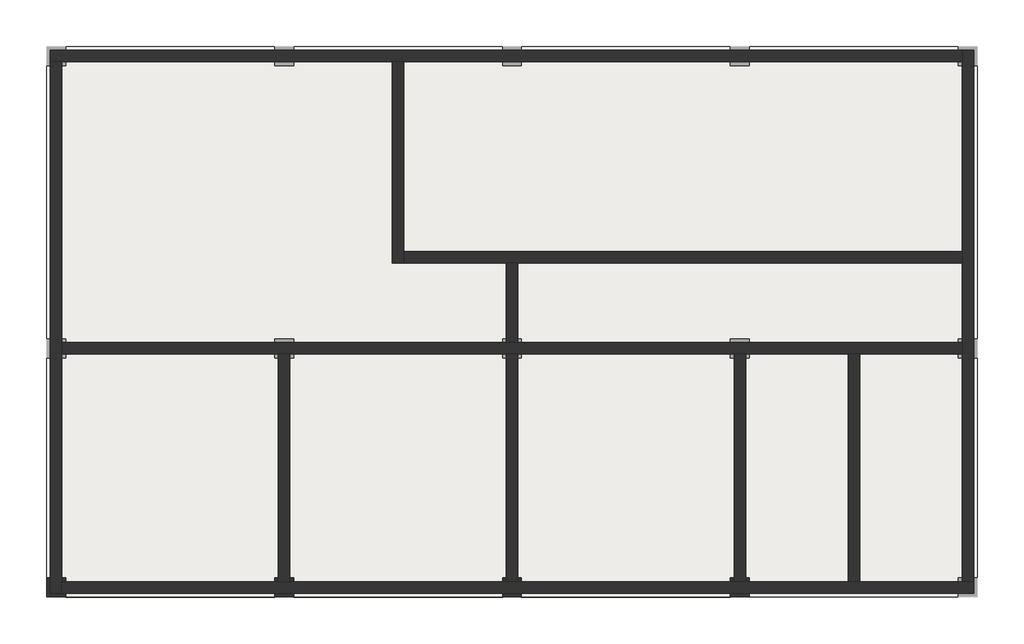
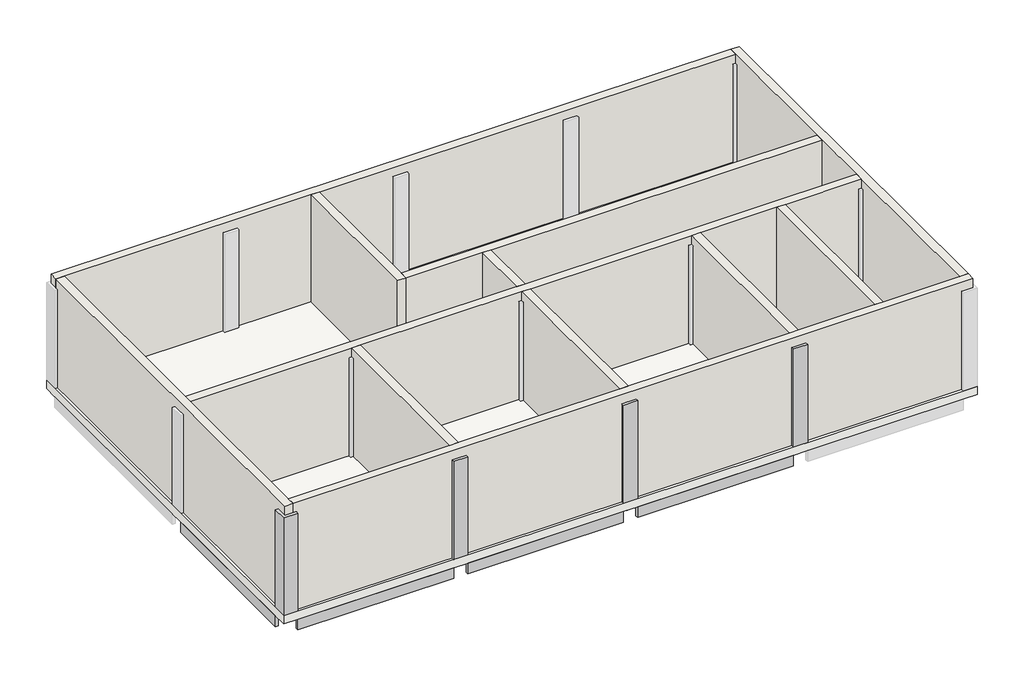
# One storey, part 1 of 2: 12 walls, 7 beams, 4 columns, 1 slab.
"""IFC4 building model written with IfcOpenShell, lengths in millimetres."""

import ifcopenshell
import ifcopenshell.guid

model = None  # the IFC model being written
_history = None  # IfcOwnerHistory: only IFC2X3 demands one
_inside = {}  # id of a spatial element -> (the spatial element, [elements in it])
_under = {}  # id of a project, library or spatial element -> (it, [spatial elements below it])
_declared = {}  # id of a project -> (the project, [libraries it declares])
_typed = {}  # id of a type object -> (the type object, [elements of that type])
_made_of = {}  # id of a material, layer set ... -> (it, [elements and type objects made of it])


def new_model(schema):
    """Start an empty IFC model of exactly this schema.

    Asked for "IFC4X3", IfcOpenShell would pick the latest addendum, in which some entities
    have other attributes; the version numbers below select the first issue.
    IFC2X3 requires an IfcOwnerHistory on every rooted entity: one is made here for all.
    """
    global model, _history
    if schema == "IFC4X3":
        model = ifcopenshell.file(schema_version=(4, 3, 0, 0))
    else:
        model = ifcopenshell.file(schema=schema)
    _inside.clear()
    _under.clear()
    _declared.clear()
    _typed.clear()
    _made_of.clear()
    _history = None
    if model.schema == "IFC2X3":
        org = make("IfcOrganization", Name="unknown")
        user = make(
            "IfcPersonAndOrganization",
            ThePerson=make("IfcPerson", FamilyName="unknown"),
            TheOrganization=org,
        )
        app = make(
            "IfcApplication",
            ApplicationDeveloper=org,
            Version="unknown",
            ApplicationFullName="unknown",
            ApplicationIdentifier="unknown",
        )
        _history = make(
            "IfcOwnerHistory",
            OwningUser=user,
            OwningApplication=app,
            ChangeAction="ADDED",
            CreationDate=0,
        )
    return model


def make(cls, **values):
    """One entity of the class cls with the attributes given. An attribute that is None is left unset."""
    return model.create_entity(
        cls, **{name: value for name, value in values.items() if value is not None}
    )


def rooted(cls, **values):
    """An entity with a GlobalId (a new one), such as an element, a storey or a relation."""
    return make(cls, GlobalId=ifcopenshell.guid.new(), OwnerHistory=_history, **values)


def si_unit(unit_type, name, prefix=None):
    """IfcSIUnit, for example si_unit("LENGTHUNIT", "METRE", prefix="MILLI")."""
    return make("IfcSIUnit", UnitType=unit_type, Prefix=prefix, Name=name)


def assignment(units):
    """IfcUnitAssignment: the units of a project."""
    return None if units is None else make("IfcUnitAssignment", Units=units)


def point(xyz):
    """IfcCartesianPoint."""
    return None if xyz is None else make("IfcCartesianPoint", Coordinates=xyz)


def direction(xyz):
    """IfcDirection."""
    return None if xyz is None else make("IfcDirection", DirectionRatios=xyz)


def frame(location, z_axis=None, x_axis=None):
    """IfcAxis2Placement3D, a coordinate frame: its origin and axes. An axis left out is left unset."""
    return make(
        "IfcAxis2Placement3D",
        Location=point(location),
        Axis=direction(z_axis),
        RefDirection=direction(x_axis),
    )


def origin():
    """The frame at (0, 0, 0) with its axes left unset."""
    return frame((0.0, 0.0, 0.0))


def place(relative_to, where):
    """IfcLocalPlacement: puts the frame where relative to a parent placement (None: the world)."""
    return make(
        "IfcLocalPlacement", PlacementRelTo=relative_to, RelativePlacement=where
    )


def context(
    kind, dimensions, precision=None, world=None, true_north=None, identifier=None
):
    """IfcGeometricRepresentationContext, for example the 3D "Model" context."""
    return make(
        "IfcGeometricRepresentationContext",
        ContextIdentifier=identifier,
        ContextType=kind,
        CoordinateSpaceDimension=dimensions,
        Precision=precision,
        WorldCoordinateSystem=world,
        TrueNorth=true_north,
    )


def project(units=None, contexts=None):
    """IfcProject with its units and contexts."""
    return rooted(
        "IfcProject",
        Name="project",
        RepresentationContexts=contexts,
        UnitsInContext=assignment(units),
    )


def spatial(cls, under=None, at=None, **own):
    """A site, building, storey or space (cls), placed at a placement, below another one or the project."""
    s = rooted(cls, ObjectPlacement=at, **own)
    if under is not None:
        _under.setdefault(under.id(), (under, []))[1].append(s)
    return s


def polyline(points):
    """IfcPolyline through the points."""
    return make("IfcPolyline", Points=[point(p) for p in points])


def outline(outer, holes=None, kind="AREA"):
    """IfcArbitraryClosedProfileDef: a profile drawn as a closed curve; with holes, ...WithVoids."""
    if holes is None:
        return make("IfcArbitraryClosedProfileDef", ProfileType=kind, OuterCurve=outer)
    return make(
        "IfcArbitraryProfileDefWithVoids",
        ProfileType=kind,
        OuterCurve=outer,
        InnerCurves=holes,
    )


def extrude(swept, where, along, depth):
    """IfcExtrudedAreaSolid: the profile swept, set in the frame where, extruded along a direction by depth."""
    return make(
        "IfcExtrudedAreaSolid",
        SweptArea=swept,
        Position=where,
        ExtrudedDirection=direction(along),
        Depth=depth,
    )


def faces_of(points, faces, orient=None, outer=None):
    """IfcFace entities. A face is a list of loops; a loop is a list of indices into points, from 0.

    orient and outer hold one flag for each loop. By default every Orientation is true, the
    first loop of a face is its IfcFaceOuterBound and the others are IfcFaceBound.
    """
    made = []
    for i, loops in enumerate(faces):
        bounds = []
        for j, loop in enumerate(loops):
            is_outer = j == 0 if outer is None else outer[i][j]
            bounds.append(
                make(
                    "IfcFaceOuterBound" if is_outer else "IfcFaceBound",
                    Bound=make("IfcPolyLoop", Polygon=[points[k] for k in loop]),
                    Orientation=True if orient is None else orient[i][j],
                )
            )
        made.append(make("IfcFace", Bounds=bounds))
    return made


def faceted_brep(points, faces, orient=None, outer=None, voids=None):
    """IfcFacetedBrep: a solid bounded by flat faces; with voids (closed shells), ...WithVoids."""
    shared = [point(p) for p in points]
    hull = make("IfcClosedShell", CfsFaces=faces_of(shared, faces, orient, outer))
    if voids is None:
        return make("IfcFacetedBrep", Outer=hull)
    return make(
        "IfcFacetedBrepWithVoids",
        Outer=hull,
        Voids=[
            make(cls, CfsFaces=faces_of(shared, fs, o, b)) for cls, fs, o, b in voids
        ],
    )


def shape(context_of_items, identifier, shape_type, items):
    """IfcShapeRepresentation: the items that make up one representation, for example the "Body"."""
    return make(
        "IfcShapeRepresentation",
        ContextOfItems=context_of_items,
        RepresentationIdentifier=identifier,
        RepresentationType=shape_type,
        Items=items,
    )


def made_of(thing, what):
    """Note that an element or type object is made of a material, layer set ...; save() writes the relation."""
    if what is not None:
        _made_of.setdefault(what.id(), (what, []))[1].append(thing)
    return thing


def element(
    cls,
    number,
    at=None,
    inside=None,
    cuts=None,
    type_object=None,
    material=None,
    context=None,
    identifier="Body",
    shape_type=None,
    held_by="IfcProductDefinitionShape",
    body=None,
    shapes=None,
    **own,
):
    """One element of the class cls, such as IfcWall. Its Tag is "e" and its number.

    at: its placement. inside: the storey or other place that contains it. cuts: it is an
    opening in that element (IfcRelVoidsElement). A single representation is given by context,
    identifier, shape_type and body (its items); several are given by shapes. held_by: the class
    of the entity that holds the representations. save() writes the other relations.
    """
    e = rooted(cls, Tag="e%d" % number, ObjectPlacement=at, **own)
    if body is not None:
        shapes = [shape(context, identifier, shape_type, body)]
    if shapes is not None:
        e.Representation = make(held_by, Representations=shapes)
    if inside is not None:
        _inside.setdefault(inside.id(), (inside, []))[1].append(e)
    if cuts is not None:
        rooted(
            "IfcRelVoidsElement", RelatingBuildingElement=cuts, RelatedOpeningElement=e
        )
    if type_object is not None:
        _typed.setdefault(type_object.id(), (type_object, []))[1].append(e)
    return made_of(e, material)


def aggregate(whole, parts):
    """IfcRelAggregates: a whole, such as a stair, and the parts it consists of."""
    return rooted("IfcRelAggregates", RelatingObject=whole, RelatedObjects=parts)


def save(model, path):
    """Write the relations noted so far, then the file.

    IfcRelAggregates (storeys below a building ...), IfcRelContainedInSpatialStructure (elements
    in a storey), IfcRelDefinesByType, IfcRelAssociatesMaterial and IfcRelDeclares: one each for
    every whole, place, type object, material and project.
    """
    for whole, parts in _under.values():
        aggregate(whole, parts)
    for where, things in _inside.values():
        rooted(
            "IfcRelContainedInSpatialStructure",
            RelatedElements=things,
            RelatingStructure=where,
        )
    for kind, things in _typed.values():
        rooted("IfcRelDefinesByType", RelatedObjects=things, RelatingType=kind)
    for what, things in _made_of.values():
        rooted("IfcRelAssociatesMaterial", RelatedObjects=things, RelatingMaterial=what)
    for by, libraries in _declared.values():
        rooted("IfcRelDeclares", RelatingContext=by, RelatedDefinitions=libraries)
    model.write(path)


model = new_model("IFC4")

# Units and contexts
model_context = context("Model", 3, world=origin())
ifc_project = project(units=[si_unit("LENGTHUNIT", "METRE", prefix="MILLI")], contexts=[model_context])

# Site, building, storey
site = spatial("IfcSite", under=ifc_project)
building = spatial("IfcBuilding", under=site)
storey = spatial("IfcBuildingStorey", under=building, Name="2nd FL GL+6,200", Elevation=6000.0)

# Beams
placement = place(None, origin())
element("IfcBeam", 1, ObjectType="RC Beam_Rectangular : 350 x 700mm", at=placement, inside=storey, context=model_context, shape_type="SweptSolid", body=[
    extrude(outline(polyline([(-18945.7273237, -4314.0236875), (-18945.7273237, 1485.9763125), (-18845.7273237, 1485.9763125), (-18845.7273237, -4314.0236875), (-18945.7273237, -4314.0236875)])), frame((0.0, 0.0, 5300.0), z_axis=(0.0, 0.0, 1.0), x_axis=(1.0, 0.0, 0.0)), (0.0, 0.0, 1.0), 400.0),
])
element("IfcBeam", 2, ObjectType="RC Beam_Rectangular : 350 x 700mm", at=placement, inside=storey, context=model_context, shape_type="SweptSolid", body=[
    extrude(outline(polyline([(-12520.7273237, 1485.9763125), (-12520.7273237, -4314.0236875), (-12545.7273237, -4314.0236875), (-12545.7273237, 1485.9763125), (-12520.7273237, 1485.9763125)])), frame((0.0, 0.0, 5300.0), z_axis=(0.0, 0.0, 1.0), x_axis=(1.0, 0.0, 0.0)), (0.0, 0.0, 1.0), 400.0),
    extrude(outline(polyline([(-12870.7273237, -4314.0236875), (-12870.7273237, 1485.9763125), (-12845.7273237, 1485.9763125), (-12845.7273237, -4314.0236875), (-12870.7273237, -4314.0236875)])), frame((0.0, 0.0, 5300.0), z_axis=(0.0, 0.0, 1.0), x_axis=(1.0, 0.0, 0.0)), (0.0, 0.0, 1.0), 400.0),
])
element("IfcBeam", 3, ObjectType="RC Beam_Rectangular : 350 x 700mm", at=placement, inside=storey, context=model_context, shape_type="SweptSolid", body=[
    extrude(outline(polyline([(-6520.7273237, 1485.9763125), (-6520.7273237, -4314.0236875), (-6545.7273237, -4314.0236875), (-6545.7273237, 1485.9763125), (-6520.7273237, 1485.9763125)])), frame((0.0, 0.0, 5300.0), z_axis=(0.0, 0.0, 1.0), x_axis=(1.0, 0.0, 0.0)), (0.0, 0.0, 1.0), 400.0),
    extrude(outline(polyline([(-6870.7273237, -4314.0236875), (-6870.7273237, 1485.9763125), (-6845.7273237, 1485.9763125), (-6845.7273237, -4314.0236875), (-6870.7273237, -4314.0236875)])), frame((0.0, 0.0, 5300.0), z_axis=(0.0, 0.0, 1.0), x_axis=(1.0, 0.0, 0.0)), (0.0, 0.0, 1.0), 400.0),
])
element("IfcBeam", 4, ObjectType="RC Beam_Rectangular : 350 x 700mm", at=placement, inside=storey, context=model_context, shape_type="SweptSolid", body=[
    extrude(outline(polyline([(-520.7273237, 1485.9763125), (-520.7273237, -4314.0236875), (-545.7273237, -4314.0236875), (-545.7273237, 1485.9763125), (-520.7273237, 1485.9763125)])), frame((0.0, 0.0, 5300.0), z_axis=(0.0, 0.0, 1.0), x_axis=(1.0, 0.0, 0.0)), (0.0, 0.0, 1.0), 400.0),
    extrude(outline(polyline([(-870.7273237, -4314.0236875), (-870.7273237, 1485.9763125), (-845.7273237, 1485.9763125), (-845.7273237, -4314.0236875), (-870.7273237, -4314.0236875)])), frame((0.0, 0.0, 5300.0), z_axis=(0.0, 0.0, 1.0), x_axis=(1.0, 0.0, 0.0)), (0.0, 0.0, 1.0), 400.0),
])
element("IfcBeam", 5, ObjectType="RC Beam_Rectangular : 350 x 700mm", at=placement, inside=storey, context=model_context, shape_type="SweptSolid", body=[
    extrude(outline(polyline([(-12945.7273237, -4814.0236875), (-18445.7273237, -4814.0236875), (-18445.7273237, -4714.0236875), (-12945.7273237, -4714.0236875), (-12945.7273237, -4814.0236875)])), frame((0.0, 0.0, 5300.0), z_axis=(0.0, 0.0, 1.0), x_axis=(1.0, 0.0, 0.0)), (0.0, 0.0, 1.0), 400.0),
])
element("IfcBeam", 6, ObjectType="RC Beam_Rectangular : 350 x 700mm", at=placement, inside=storey, context=model_context, shape_type="SweptSolid", body=[
    extrude(outline(polyline([(-6945.7273237, -4714.0236875), (-6945.7273237, -4814.0236875), (-12445.7273237, -4814.0236875), (-12445.7273237, -4714.0236875), (-6945.7273237, -4714.0236875)])), frame((0.0, 0.0, 5300.0), z_axis=(0.0, 0.0, 1.0), x_axis=(1.0, 0.0, 0.0)), (0.0, 0.0, 1.0), 400.0),
])
element("IfcBeam", 7, ObjectType="RC Beam_Rectangular : 350 x 700mm", at=placement, inside=storey, context=model_context, shape_type="SweptSolid", body=[
    extrude(outline(polyline([(-945.7273237, -4714.0236875), (-945.7273237, -4814.0236875), (-6445.7273237, -4814.0236875), (-6445.7273237, -4714.0236875), (-945.7273237, -4714.0236875)])), frame((0.0, 0.0, 5300.0), z_axis=(0.0, 0.0, 1.0), x_axis=(1.0, 0.0, 0.0)), (0.0, 0.0, 1.0), 400.0),
])

# Columns
element("IfcColumn", 8, ObjectType="RC_Column_Rectangular : 500 x 500mm", at=placement, inside=storey, context=model_context, shape_type="Brep", body=[
    faceted_brep([(-18545.7273237, -4314.0236875, 6000.0), (-18445.7273237, -4314.0236875, 6000.0), (-18445.7273237, -4414.0236875, 6000.0), (-18545.7273237, -4414.0236875, 6000.0), (-18445.7273237, -4314.0236875, 9667.0), (-18545.7273237, -4314.0236875, 9667.0), (-18445.7273237, -4414.0236875, 9667.0), (-18545.7273237, -4414.0236875, 9667.0)], [[[0, 1, 2, 3]], [[4, 1, 0, 5]], [[1, 4, 6, 2]], [[5, 0, 3, 7]], [[3, 2, 6, 7]], [[4, 5, 7, 6]]]),
    faceted_brep([(-18945.7273237, -4314.0236875, 6000.0), (-18945.7273237, -4814.0236875, 6000.0), (-18945.7273237, -4814.0236875, 9667.0), (-18945.7273237, -4314.0236875, 9667.0), (-18945.7273237, -4314.0236875, 9300.0), (-18445.7273237, -4814.0236875, 6000.0), (-18445.7273237, -4814.0236875, 9300.0), (-18445.7273237, -4814.0236875, 9667.0), (-18445.7273237, -4714.0236875, 9667.0), (-18845.7273237, -4714.0236875, 9667.0), (-18845.7273237, -4314.0236875, 9667.0), (-18845.7273237, -4714.0236875, 6000.0), (-18845.7273237, -4314.0236875, 6000.0), (-18845.7273237, -4314.0236875, 9300.0), (-18445.7273237, -4714.0236875, 9300.0), (-18445.7273237, -4714.0236875, 6000.0), (-18545.7273237, -4714.0236875, 6000.0)], [[[0, 1, 2, 3, 4]], [[1, 5, 6, 7, 2]], [[3, 2, 7, 8, 9, 10]], [[9, 11, 12, 13, 10]], [[11, 9, 8, 14, 15, 16]], [[0, 4, 3, 10, 13, 12]], [[5, 1, 0, 12, 11, 16, 15]], [[7, 6, 5, 15, 14, 8]]]),
])
element("IfcColumn", 9, ObjectType="RC_Column_Rectangular : 500 x 500mm", at=placement, inside=storey, context=model_context, shape_type="Brep", body=[
    faceted_brep([(-12945.7273237, -4414.0236875, 6000.0), (-12945.7273237, -4314.0236875, 6000.0), (-12845.7273237, -4314.0236875, 6000.0), (-12845.7273237, -4414.0236875, 6000.0), (-12945.7273237, -4314.0236875, 9667.0), (-12945.7273237, -4414.0236875, 9667.0), (-12845.7273237, -4414.0236875, 9667.0), (-12845.7273237, -4314.0236875, 9667.0), (-12870.7273237, -4314.0236875, 9667.0), (-12845.7273237, -4314.0236875, 9300.0)], [[[0, 1, 2, 3]], [[4, 1, 0, 5]], [[4, 5, 6, 7, 8]], [[3, 2, 9, 7, 6]], [[1, 4, 8, 7, 9, 2]], [[5, 0, 3, 6]]]),
    faceted_brep([(-12445.7273237, -4314.0236875, 9667.0), (-12445.7273237, -4314.0236875, 6000.0), (-12545.7273237, -4314.0236875, 6000.0), (-12545.7273237, -4314.0236875, 9300.0), (-12545.7273237, -4314.0236875, 9667.0), (-12520.7273237, -4314.0236875, 9667.0), (-12445.7273237, -4414.0236875, 9667.0), (-12445.7273237, -4414.0236875, 6000.0), (-12545.7273237, -4414.0236875, 9667.0), (-12545.7273237, -4414.0236875, 6000.0)], [[[0, 1, 2, 3, 4, 5]], [[1, 0, 6, 7]], [[7, 6, 8, 9]], [[2, 9, 8, 4, 3]], [[1, 7, 9, 2]], [[6, 0, 5, 4, 8]]]),
    faceted_brep([(-12945.7273237, -4814.0236875, 6000.0), (-12445.7273237, -4814.0236875, 6000.0), (-12445.7273237, -4814.0236875, 9300.0), (-12445.7273237, -4814.0236875, 9667.0), (-12945.7273237, -4814.0236875, 9667.0), (-12945.7273237, -4814.0236875, 9300.0), (-12445.7273237, -4714.0236875, 6000.0), (-12945.7273237, -4714.0236875, 6000.0), (-12945.7273237, -4714.0236875, 9300.0), (-12945.7273237, -4714.0236875, 9667.0), (-12445.7273237, -4714.0236875, 9667.0), (-12445.7273237, -4714.0236875, 9300.0)], [[[0, 1, 2, 3, 4, 5]], [[6, 7, 8, 9, 10, 11]], [[1, 0, 7, 6]], [[0, 5, 4, 9, 8, 7]], [[3, 2, 1, 6, 11, 10]], [[4, 3, 10, 9]]]),
])
element("IfcColumn", 10, ObjectType="RC_Column_Rectangular : 500 x 500mm", at=placement, inside=storey, context=model_context, shape_type="Brep", body=[
    faceted_brep([(-6945.7273237, -4414.0236875, 6000.0), (-6945.7273237, -4314.0236875, 6000.0), (-6845.7273237, -4314.0236875, 6000.0), (-6845.7273237, -4414.0236875, 6000.0), (-6945.7273237, -4314.0236875, 9667.0), (-6945.7273237, -4414.0236875, 9667.0), (-6845.7273237, -4414.0236875, 9667.0), (-6845.7273237, -4314.0236875, 9667.0), (-6870.7273237, -4314.0236875, 9667.0), (-6845.7273237, -4314.0236875, 9300.0)], [[[0, 1, 2, 3]], [[4, 1, 0, 5]], [[4, 5, 6, 7, 8]], [[3, 2, 9, 7, 6]], [[1, 4, 8, 7, 9, 2]], [[5, 0, 3, 6]]]),
    faceted_brep([(-6445.7273237, -4314.0236875, 9667.0), (-6445.7273237, -4314.0236875, 6000.0), (-6545.7273237, -4314.0236875, 6000.0), (-6545.7273237, -4314.0236875, 9300.0), (-6545.7273237, -4314.0236875, 9667.0), (-6520.7273237, -4314.0236875, 9667.0), (-6445.7273237, -4414.0236875, 9667.0), (-6445.7273237, -4414.0236875, 6000.0), (-6545.7273237, -4414.0236875, 9667.0), (-6545.7273237, -4414.0236875, 6000.0)], [[[0, 1, 2, 3, 4, 5]], [[1, 0, 6, 7]], [[7, 6, 8, 9]], [[2, 9, 8, 4, 3]], [[1, 7, 9, 2]], [[6, 0, 5, 4, 8]]]),
    faceted_brep([(-6945.7273237, -4814.0236875, 6000.0), (-6445.7273237, -4814.0236875, 6000.0), (-6445.7273237, -4814.0236875, 9300.0), (-6445.7273237, -4814.0236875, 9667.0), (-6945.7273237, -4814.0236875, 9667.0), (-6945.7273237, -4814.0236875, 9300.0), (-6445.7273237, -4714.0236875, 6000.0), (-6945.7273237, -4714.0236875, 6000.0), (-6945.7273237, -4714.0236875, 9300.0), (-6945.7273237, -4714.0236875, 9667.0), (-6445.7273237, -4714.0236875, 9667.0), (-6445.7273237, -4714.0236875, 9300.0)], [[[0, 1, 2, 3, 4, 5]], [[6, 7, 8, 9, 10, 11]], [[1, 0, 7, 6]], [[0, 5, 4, 9, 8, 7]], [[3, 2, 1, 6, 11, 10]], [[4, 3, 10, 9]]]),
])
element("IfcColumn", 11, ObjectType="RC_Column_Rectangular : 500 x 500mm", at=placement, inside=storey, context=model_context, shape_type="Brep", body=[
    faceted_brep([(-945.7273237, -4414.0236875, 6000.0), (-945.7273237, -4314.0236875, 6000.0), (-845.7273237, -4314.0236875, 6000.0), (-845.7273237, -4414.0236875, 6000.0), (-945.7273237, -4314.0236875, 9667.0), (-945.7273237, -4414.0236875, 9667.0), (-845.7273237, -4414.0236875, 9667.0), (-845.7273237, -4314.0236875, 9667.0), (-870.7273237, -4314.0236875, 9667.0), (-845.7273237, -4314.0236875, 9300.0)], [[[0, 1, 2, 3]], [[4, 1, 0, 5]], [[4, 5, 6, 7, 8]], [[3, 2, 9, 7, 6]], [[1, 4, 8, 7, 9, 2]], [[5, 0, 3, 6]]]),
    faceted_brep([(-445.7273237, -4314.0236875, 9667.0), (-445.7273237, -4314.0236875, 6000.0), (-545.7273237, -4314.0236875, 6000.0), (-545.7273237, -4314.0236875, 9300.0), (-545.7273237, -4314.0236875, 9667.0), (-520.7273237, -4314.0236875, 9667.0), (-445.7273237, -4414.0236875, 9667.0), (-445.7273237, -4414.0236875, 6000.0), (-545.7273237, -4414.0236875, 9667.0), (-545.7273237, -4414.0236875, 6000.0)], [[[0, 1, 2, 3, 4, 5]], [[1, 0, 6, 7]], [[7, 6, 8, 9]], [[2, 9, 8, 4, 3]], [[1, 7, 9, 2]], [[6, 0, 5, 4, 8]]]),
    faceted_brep([(-945.7273237, -4814.0236875, 6000.0), (-445.7273237, -4814.0236875, 6000.0), (-445.7273237, -4814.0236875, 9667.0), (-945.7273237, -4814.0236875, 9667.0), (-945.7273237, -4814.0236875, 9300.0), (-445.7273237, -4714.0236875, 6000.0), (-945.7273237, -4714.0236875, 6000.0), (-945.7273237, -4714.0236875, 9300.0), (-945.7273237, -4714.0236875, 9667.0), (-445.7273237, -4714.0236875, 9667.0)], [[[0, 1, 2, 3, 4]], [[5, 6, 7, 8, 9]], [[1, 0, 6, 5]], [[0, 4, 3, 8, 7, 6]], [[2, 1, 5, 9]], [[3, 2, 9, 8]]]),
])

# Slab
element("IfcSlab", 12, ObjectType="H_FL_ACS_RC Slab_T150", at=placement, inside=storey, context=model_context, shape_type="Brep", body=[
    faceted_brep([(5554.2726763, -4814.0236875, 5700.0), (5054.2726763, -4814.0236875, 5700.0), (-445.7273237, -4814.0236875, 5700.0), (-945.7273237, -4814.0236875, 5700.0), (-6445.7273237, -4814.0236875, 5700.0), (-6945.7273237, -4814.0236875, 5700.0), (-12445.7273237, -4814.0236875, 5700.0), (-12945.7273237, -4814.0236875, 5700.0), (-18445.7273237, -4814.0236875, 5700.0), (-18945.7273237, -4814.0236875, 5700.0), (-18945.7273237, -4314.0236875, 5700.0), (-18945.7273237, 1485.9763125, 5700.0), (-18945.7273237, 1985.9763125, 5700.0), (-18945.7273237, 9185.9763125, 5700.0), (-18945.7273237, 9685.9763125, 5700.0), (-18445.7273237, 9685.9763125, 5700.0), (-12945.7273237, 9685.9763125, 5700.0), (-12445.7273237, 9685.9763125, 5700.0), (-12433.0273237, 9685.9763125, 5700.0), (-6945.7273237, 9685.9763125, 5700.0), (-6445.7273237, 9685.9763125, 5700.0), (-6433.0273237, 9685.9763125, 5700.0), (-945.7273237, 9685.9763125, 5700.0), (-445.7273237, 9685.9763125, 5700.0), (-433.0273237, 9685.9763125, 5700.0), (5054.2726763, 9685.9763125, 5700.0), (5554.2726763, 9685.9763125, 5700.0), (5554.2726763, 9185.9763125, 5700.0), (5554.2726763, 1998.6763125, 5700.0), (5554.2726763, 1985.9763125, 5700.0), (5554.2726763, 1485.9763125, 5700.0), (5554.2726763, -4314.0236875, 5700.0), (5554.2726763, -4814.0236875, 6000.0), (5554.2726763, 9685.9763125, 6000.0), (-18945.7273237, 9685.9763125, 6000.0), (-18945.7273237, -4814.0236875, 6000.0)], [[[0, 1, 2, 3, 4, 5, 6, 7, 8, 9, 10, 11, 12, 13, 14, 15, 16, 17, 18, 19, 20, 21, 22, 23, 24, 25, 26, 27, 28, 29, 30, 31]], [[32, 33, 34, 35]], [[9, 8, 7, 6, 5, 4, 3, 2, 1, 0, 32, 35]], [[14, 13, 12, 11, 10, 9, 35, 34]], [[26, 25, 24, 23, 22, 21, 20, 19, 18, 17, 16, 15, 14, 34, 33]], [[0, 31, 30, 29, 28, 27, 26, 33, 32]]]),
])

# Walls
element("IfcWall", 13, ObjectType="일반 - 300mm", at=placement, inside=storey, context=model_context, shape_type="Brep", body=[
    faceted_brep([(-18845.7273237, 9285.9763125, 6000.0), (-18545.7273237, 9285.9763125, 6000.0), (-18445.7273237, 9285.9763125, 6000.0), (-12945.7273237, 9285.9763125, 6000.0), (-12445.7273237, 9285.9763125, 6000.0), (-9845.7273237, 9285.9763125, 6000.0), (-9545.7273237, 9285.9763125, 6000.0), (-6945.7273237, 9285.9763125, 6000.0), (-6445.7273237, 9285.9763125, 6000.0), (-945.7273237, 9285.9763125, 6000.0), (-445.7273237, 9285.9763125, 6000.0), (5054.2726763, 9285.9763125, 6000.0), (5154.2726763, 9285.9763125, 6000.0), (5154.2726763, 9285.9763125, 9667.0), (5154.2726763, 9285.9763125, 10000.0), (-9545.7273237, 9285.9763125, 10000.0), (-9845.7273237, 9285.9763125, 10000.0), (-18545.7273237, 9285.9763125, 10000.0), (-18845.7273237, 9285.9763125, 10000.0), (-18845.7273237, 9585.9763125, 6000.0), (-18845.7273237, 9585.9763125, 9667.0), (-18845.7273237, 9585.9763125, 10000.0), (5154.2726763, 9585.9763125, 10000.0), (5154.2726763, 9585.9763125, 6000.0), (5054.2726763, 9585.9763125, 6000.0), (-445.7273237, 9585.9763125, 6000.0), (-945.7273237, 9585.9763125, 6000.0), (-6445.7273237, 9585.9763125, 6000.0), (-6945.7273237, 9585.9763125, 6000.0), (-12445.7273237, 9585.9763125, 6000.0), (-12945.7273237, 9585.9763125, 6000.0), (-18445.7273237, 9585.9763125, 6000.0)], [[[0, 1, 2, 3, 4, 5, 6, 7, 8, 9, 10, 11, 12, 13, 14, 15, 16, 17, 18]], [[19, 20, 21, 22, 23, 24, 25, 26, 27, 28, 29, 30, 31]], [[12, 11, 10, 9, 8, 7, 6, 5, 4, 3, 2, 1, 0, 19, 31, 30, 29, 28, 27, 26, 25, 24, 23]], [[18, 17, 16, 15, 14, 22, 21]], [[0, 18, 21, 20, 19]], [[14, 13, 12, 23, 22]]]),
])
element("IfcWall", 14, ObjectType="일반 - 300mm", at=placement, inside=storey, context=model_context, shape_type="Brep", body=[
    faceted_brep([(-18545.7273237, -4714.0236875, 6000.0), (-18545.7273237, -4414.0236875, 6000.0), (-18545.7273237, -4314.0236875, 6000.0), (-18545.7273237, 1485.9763125, 6000.0), (-18545.7273237, 1585.9763125, 6000.0), (-18545.7273237, 1885.9763125, 6000.0), (-18545.7273237, 1985.9763125, 6000.0), (-18545.7273237, 9185.9763125, 6000.0), (-18545.7273237, 9285.9763125, 6000.0), (-18545.7273237, 9285.9763125, 9667.0), (-18545.7273237, 9285.9763125, 10000.0), (-18545.7273237, 1885.9763125, 10000.0), (-18545.7273237, 1585.9763125, 10000.0), (-18545.7273237, -4414.0236875, 10000.0), (-18545.7273237, -4714.0236875, 10000.0), (-18845.7273237, -4714.0236875, 6000.0), (-18845.7273237, -4714.0236875, 9667.0), (-18845.7273237, -4714.0236875, 10000.0), (-18845.7273237, 9285.9763125, 10000.0), (-18845.7273237, 9285.9763125, 6000.0), (-18845.7273237, 9185.9763125, 6000.0), (-18845.7273237, 1985.9763125, 6000.0), (-18845.7273237, 1485.9763125, 6000.0), (-18845.7273237, -4314.0236875, 6000.0)], [[[0, 1, 2, 3, 4, 5, 6, 7, 8, 9, 10, 11, 12, 13, 14]], [[15, 16, 17, 18, 19, 20, 21, 22, 23]], [[8, 7, 6, 5, 4, 3, 2, 1, 0, 15, 23, 22, 21, 20, 19]], [[14, 13, 12, 11, 10, 18, 17]], [[0, 14, 17, 16, 15]], [[10, 9, 8, 19, 18]]]),
])
element("IfcWall", 15, ObjectType="일반 - 300mm", at=placement, inside=storey, context=model_context, shape_type="Brep", body=[
    faceted_brep([(5454.2726763, -4414.0236875, 6000.0), (5154.2726763, -4414.0236875, 6000.0), (5054.2726763, -4414.0236875, 6000.0), (2454.2726763, -4414.0236875, 6000.0), (2154.2726763, -4414.0236875, 6000.0), (-445.7273237, -4414.0236875, 6000.0), (-545.7273237, -4414.0236875, 6000.0), (-845.7273237, -4414.0236875, 6000.0), (-945.7273237, -4414.0236875, 6000.0), (-6445.7273237, -4414.0236875, 6000.0), (-6545.7273237, -4414.0236875, 6000.0), (-6845.7273237, -4414.0236875, 6000.0), (-6945.7273237, -4414.0236875, 6000.0), (-12445.7273237, -4414.0236875, 6000.0), (-12545.7273237, -4414.0236875, 6000.0), (-12845.7273237, -4414.0236875, 6000.0), (-12945.7273237, -4414.0236875, 6000.0), (-18445.7273237, -4414.0236875, 6000.0), (-18545.7273237, -4414.0236875, 6000.0), (-18545.7273237, -4414.0236875, 9667.0), (-18545.7273237, -4414.0236875, 10000.0), (-12845.7273237, -4414.0236875, 10000.0), (-12545.7273237, -4414.0236875, 10000.0), (-6845.7273237, -4414.0236875, 10000.0), (-6545.7273237, -4414.0236875, 10000.0), (-845.7273237, -4414.0236875, 10000.0), (-545.7273237, -4414.0236875, 10000.0), (2154.2726763, -4414.0236875, 10000.0), (2454.2726763, -4414.0236875, 10000.0), (5154.2726763, -4414.0236875, 10000.0), (5454.2726763, -4414.0236875, 10000.0), (5454.2726763, -4714.0236875, 6000.0), (5454.2726763, -4714.0236875, 9667.0), (5454.2726763, -4714.0236875, 10000.0), (-18545.7273237, -4714.0236875, 10000.0), (-18545.7273237, -4714.0236875, 6000.0), (-18445.7273237, -4714.0236875, 6000.0), (-12945.7273237, -4714.0236875, 6000.0), (-12445.7273237, -4714.0236875, 6000.0), (-6945.7273237, -4714.0236875, 6000.0), (-6445.7273237, -4714.0236875, 6000.0), (-945.7273237, -4714.0236875, 6000.0), (-445.7273237, -4714.0236875, 6000.0), (5054.2726763, -4714.0236875, 6000.0)], [[[0, 1, 2, 3, 4, 5, 6, 7, 8, 9, 10, 11, 12, 13, 14, 15, 16, 17, 18, 19, 20, 21, 22, 23, 24, 25, 26, 27, 28, 29, 30]], [[31, 32, 33, 34, 35, 36, 37, 38, 39, 40, 41, 42, 43]], [[18, 17, 16, 15, 14, 13, 12, 11, 10, 9, 8, 7, 6, 5, 4, 3, 2, 1, 0, 31, 43, 42, 41, 40, 39, 38, 37, 36, 35]], [[30, 29, 28, 27, 26, 25, 24, 23, 22, 21, 20, 34, 33]], [[0, 30, 33, 32, 31]], [[20, 19, 18, 35, 34]]]),
])
element("IfcWall", 16, ObjectType="일반 - 300mm", at=placement, inside=storey, context=model_context, shape_type="Brep", body=[
    faceted_brep([(5154.2726763, 9585.9763125, 6000.0), (5154.2726763, 9285.9763125, 6000.0), (5154.2726763, 9185.9763125, 6000.0), (5154.2726763, 4285.9763125, 6000.0), (5154.2726763, 3985.9763125, 6000.0), (5154.2726763, 1985.9763125, 6000.0), (5154.2726763, 1885.9763125, 6000.0), (5154.2726763, 1585.9763125, 6000.0), (5154.2726763, 1485.9763125, 6000.0), (5154.2726763, -4314.0236875, 6000.0), (5154.2726763, -4414.0236875, 6000.0), (5154.2726763, -4414.0236875, 9667.0), (5154.2726763, -4414.0236875, 10000.0), (5154.2726763, 1585.9763125, 10000.0), (5154.2726763, 1885.9763125, 10000.0), (5154.2726763, 3985.9763125, 10000.0), (5154.2726763, 4285.9763125, 10000.0), (5154.2726763, 9285.9763125, 10000.0), (5154.2726763, 9585.9763125, 10000.0), (5454.2726763, 9585.9763125, 6000.0), (5454.2726763, 9585.9763125, 9667.0), (5454.2726763, 9585.9763125, 10000.0), (5454.2726763, -4414.0236875, 10000.0), (5454.2726763, -4414.0236875, 6000.0), (5454.2726763, -4314.0236875, 6000.0), (5454.2726763, 1485.9763125, 6000.0), (5454.2726763, 1985.9763125, 6000.0), (5454.2726763, 9185.9763125, 6000.0)], [[[0, 1, 2, 3, 4, 5, 6, 7, 8, 9, 10, 11, 12, 13, 14, 15, 16, 17, 18]], [[19, 20, 21, 22, 23, 24, 25, 26, 27]], [[10, 9, 8, 7, 6, 5, 4, 3, 2, 1, 0, 19, 27, 26, 25, 24, 23]], [[18, 17, 16, 15, 14, 13, 12, 22, 21]], [[0, 18, 21, 20, 19]], [[12, 11, 10, 23, 22]]]),
])
element("IfcWall", 17, ObjectType="일반 - 300mm", at=placement, inside=storey, context=model_context, shape_type="Brep", body=[
    faceted_brep([(-18545.7273237, 1585.9763125, 6000.0), (-18445.7273237, 1585.9763125, 6000.0), (-12945.7273237, 1585.9763125, 6000.0), (-12845.7273237, 1585.9763125, 6000.0), (-12545.7273237, 1585.9763125, 6000.0), (-12445.7273237, 1585.9763125, 6000.0), (-6945.7273237, 1585.9763125, 6000.0), (-6845.7273237, 1585.9763125, 6000.0), (-6545.7273237, 1585.9763125, 6000.0), (-6445.7273237, 1585.9763125, 6000.0), (-945.7273237, 1585.9763125, 6000.0), (-845.7273237, 1585.9763125, 6000.0), (-545.7273237, 1585.9763125, 6000.0), (-445.7273237, 1585.9763125, 6000.0), (2154.2726763, 1585.9763125, 6000.0), (2454.2726763, 1585.9763125, 6000.0), (5054.2726763, 1585.9763125, 6000.0), (5154.2726763, 1585.9763125, 6000.0), (5154.2726763, 1585.9763125, 9667.0), (5154.2726763, 1585.9763125, 10000.0), (2454.2726763, 1585.9763125, 10000.0), (2154.2726763, 1585.9763125, 10000.0), (-545.7273237, 1585.9763125, 10000.0), (-845.7273237, 1585.9763125, 10000.0), (-6545.7273237, 1585.9763125, 10000.0), (-6845.7273237, 1585.9763125, 10000.0), (-12545.7273237, 1585.9763125, 10000.0), (-12845.7273237, 1585.9763125, 10000.0), (-18545.7273237, 1585.9763125, 10000.0), (-18545.7273237, 1585.9763125, 9667.0), (-18545.7273237, 1885.9763125, 6000.0), (-18545.7273237, 1885.9763125, 9667.0), (-18545.7273237, 1885.9763125, 10000.0), (-6845.7273237, 1885.9763125, 10000.0), (-6545.7273237, 1885.9763125, 10000.0), (5154.2726763, 1885.9763125, 10000.0), (5154.2726763, 1885.9763125, 9667.0), (5154.2726763, 1885.9763125, 6000.0), (5054.2726763, 1885.9763125, 6000.0), (-445.7273237, 1885.9763125, 6000.0), (-945.7273237, 1885.9763125, 6000.0), (-6445.7273237, 1885.9763125, 6000.0), (-6545.7273237, 1885.9763125, 6000.0), (-6845.7273237, 1885.9763125, 6000.0), (-6945.7273237, 1885.9763125, 6000.0), (-12445.7273237, 1885.9763125, 6000.0), (-12945.7273237, 1885.9763125, 6000.0), (-18445.7273237, 1885.9763125, 6000.0)], [[[0, 1, 2, 3, 4, 5, 6, 7, 8, 9, 10, 11, 12, 13, 14, 15, 16, 17, 18, 19, 20, 21, 22, 23, 24, 25, 26, 27, 28, 29]], [[30, 31, 32, 33, 34, 35, 36, 37, 38, 39, 40, 41, 42, 43, 44, 45, 46, 47]], [[17, 16, 15, 14, 13, 12, 11, 10, 9, 8, 7, 6, 5, 4, 3, 2, 1, 0, 30, 47, 46, 45, 44, 43, 42, 41, 40, 39, 38, 37]], [[28, 27, 26, 25, 24, 23, 22, 21, 20, 19, 35, 34, 33, 32]], [[19, 18, 17, 37, 36, 35]], [[0, 29, 28, 32, 31, 30]]]),
])
element("IfcWall", 18, ObjectType="일반 - 300mm", at=placement, inside=storey, context=model_context, shape_type="Brep", body=[
    faceted_brep([(-9845.7273237, 9285.9763125, 6000.0), (-9845.7273237, 3985.9763125, 6000.0), (-9845.7273237, 3985.9763125, 10000.0), (-9845.7273237, 9285.9763125, 10000.0), (-9545.7273237, 9285.9763125, 6000.0), (-9545.7273237, 9285.9763125, 10000.0), (-9545.7273237, 4285.9763125, 10000.0), (-9545.7273237, 3985.9763125, 10000.0), (-9545.7273237, 3985.9763125, 6000.0), (-9545.7273237, 4285.9763125, 6000.0)], [[[0, 1, 2, 3]], [[4, 5, 6, 7, 8, 9]], [[1, 0, 4, 9, 8]], [[3, 2, 7, 6, 5]], [[0, 3, 5, 4]], [[2, 1, 8, 7]]]),
])
element("IfcWall", 19, ObjectType="일반 - 300mm", at=placement, inside=storey, context=model_context, shape_type="Brep", body=[
    faceted_brep([(-9545.7273237, 3985.9763125, 6000.0), (-6845.7273237, 3985.9763125, 6000.0), (-6545.7273237, 3985.9763125, 6000.0), (5154.2726763, 3985.9763125, 6000.0), (5154.2726763, 3985.9763125, 10000.0), (-6545.7273237, 3985.9763125, 10000.0), (-6845.7273237, 3985.9763125, 10000.0), (-9545.7273237, 3985.9763125, 10000.0), (-9545.7273237, 4285.9763125, 6000.0), (-9545.7273237, 4285.9763125, 10000.0), (5154.2726763, 4285.9763125, 10000.0), (5154.2726763, 4285.9763125, 6000.0)], [[[0, 1, 2, 3, 4, 5, 6, 7]], [[8, 9, 10, 11]], [[3, 2, 1, 0, 8, 11]], [[7, 6, 5, 4, 10, 9]], [[0, 7, 9, 8]], [[4, 3, 11, 10]]]),
])
element("IfcWall", 20, ObjectType="일반 - 300mm", at=placement, inside=storey, context=model_context, shape_type="Brep", body=[
    faceted_brep([(-6845.7273237, 3985.9763125, 6000.0), (-6845.7273237, 1985.9763125, 6000.0), (-6845.7273237, 1885.9763125, 6000.0), (-6845.7273237, 1885.9763125, 9667.0), (-6845.7273237, 1885.9763125, 10000.0), (-6845.7273237, 3985.9763125, 10000.0), (-6845.7273237, 3985.9763125, 9667.0), (-6845.7273237, 3985.9763125, 9300.0), (-6545.7273237, 3985.9763125, 6000.0), (-6545.7273237, 3985.9763125, 9300.0), (-6545.7273237, 3985.9763125, 9667.0), (-6545.7273237, 3985.9763125, 10000.0), (-6545.7273237, 1885.9763125, 10000.0), (-6545.7273237, 1885.9763125, 9667.0), (-6545.7273237, 1885.9763125, 6000.0), (-6545.7273237, 1985.9763125, 6000.0)], [[[0, 1, 2, 3, 4, 5, 6, 7]], [[8, 9, 10, 11, 12, 13, 14, 15]], [[2, 1, 0, 8, 15, 14]], [[5, 4, 12, 11]], [[4, 3, 2, 14, 13, 12]], [[0, 7, 6, 5, 11, 10, 9, 8]]]),
])
element("IfcWall", 21, ObjectType="일반 - 300mm", at=placement, inside=storey, context=model_context, shape_type="Brep", body=[
    faceted_brep([(2154.2726763, 1585.9763125, 6000.0), (2154.2726763, -4414.0236875, 6000.0), (2154.2726763, -4414.0236875, 10000.0), (2154.2726763, 1585.9763125, 10000.0), (2154.2726763, 1585.9763125, 9667.0), (2154.2726763, 1585.9763125, 9300.0), (2454.2726763, 1585.9763125, 6000.0), (2454.2726763, 1585.9763125, 9300.0), (2454.2726763, 1585.9763125, 9667.0), (2454.2726763, 1585.9763125, 10000.0), (2454.2726763, -4414.0236875, 10000.0), (2454.2726763, -4414.0236875, 6000.0)], [[[0, 1, 2, 3, 4, 5]], [[6, 7, 8, 9, 10, 11]], [[1, 0, 6, 11]], [[3, 2, 10, 9]], [[2, 1, 11, 10]], [[0, 5, 4, 3, 9, 8, 7, 6]]]),
])
element("IfcWall", 22, ObjectType="일반 - 300mm", at=placement, inside=storey, context=model_context, shape_type="Brep", body=[
    faceted_brep([(-6845.7273237, 1585.9763125, 6000.0), (-6845.7273237, 1485.9763125, 6000.0), (-6845.7273237, -4314.0236875, 6000.0), (-6845.7273237, -4414.0236875, 6000.0), (-6845.7273237, -4414.0236875, 9667.0), (-6845.7273237, -4414.0236875, 10000.0), (-6845.7273237, 1585.9763125, 10000.0), (-6845.7273237, 1585.9763125, 9667.0), (-6545.7273237, 1585.9763125, 6000.0), (-6545.7273237, 1585.9763125, 9667.0), (-6545.7273237, 1585.9763125, 10000.0), (-6545.7273237, -4414.0236875, 10000.0), (-6545.7273237, -4414.0236875, 9667.0), (-6545.7273237, -4414.0236875, 6000.0), (-6545.7273237, -4314.0236875, 6000.0), (-6545.7273237, 1485.9763125, 6000.0)], [[[0, 1, 2, 3, 4, 5, 6, 7]], [[8, 9, 10, 11, 12, 13, 14, 15]], [[3, 2, 1, 0, 8, 15, 14, 13]], [[6, 5, 11, 10]], [[5, 4, 3, 13, 12, 11]], [[0, 7, 6, 10, 9, 8]]]),
])
element("IfcWall", 23, ObjectType="일반 - 300mm", at=placement, inside=storey, context=model_context, shape_type="Brep", body=[
    faceted_brep([(-12845.7273237, 1585.9763125, 6000.0), (-12845.7273237, 1485.9763125, 6000.0), (-12845.7273237, -4314.0236875, 6000.0), (-12845.7273237, -4414.0236875, 6000.0), (-12845.7273237, -4414.0236875, 9667.0), (-12845.7273237, -4414.0236875, 10000.0), (-12845.7273237, 1585.9763125, 10000.0), (-12845.7273237, 1585.9763125, 9667.0), (-12545.7273237, 1585.9763125, 6000.0), (-12545.7273237, 1585.9763125, 9667.0), (-12545.7273237, 1585.9763125, 10000.0), (-12545.7273237, -4414.0236875, 10000.0), (-12545.7273237, -4414.0236875, 9667.0), (-12545.7273237, -4414.0236875, 6000.0), (-12545.7273237, -4314.0236875, 6000.0), (-12545.7273237, 1485.9763125, 6000.0)], [[[0, 1, 2, 3, 4, 5, 6, 7]], [[8, 9, 10, 11, 12, 13, 14, 15]], [[3, 2, 1, 0, 8, 15, 14, 13]], [[6, 5, 11, 10]], [[5, 4, 3, 13, 12, 11]], [[0, 7, 6, 10, 9, 8]]]),
])
element("IfcWall", 24, ObjectType="일반 - 300mm", at=placement, inside=storey, context=model_context, shape_type="Brep", body=[
    faceted_brep([(-845.7273237, 1585.9763125, 6000.0), (-845.7273237, 1485.9763125, 6000.0), (-845.7273237, -4314.0236875, 6000.0), (-845.7273237, -4414.0236875, 6000.0), (-845.7273237, -4414.0236875, 9667.0), (-845.7273237, -4414.0236875, 10000.0), (-845.7273237, 1585.9763125, 10000.0), (-845.7273237, 1585.9763125, 9667.0), (-545.7273237, 1585.9763125, 6000.0), (-545.7273237, 1585.9763125, 9667.0), (-545.7273237, 1585.9763125, 10000.0), (-545.7273237, -4414.0236875, 10000.0), (-545.7273237, -4414.0236875, 9667.0), (-545.7273237, -4414.0236875, 6000.0), (-545.7273237, -4314.0236875, 6000.0), (-545.7273237, 1485.9763125, 6000.0)], [[[0, 1, 2, 3, 4, 5, 6, 7]], [[8, 9, 10, 11, 12, 13, 14, 15]], [[3, 2, 1, 0, 8, 15, 14, 13]], [[6, 5, 11, 10]], [[5, 4, 3, 13, 12, 11]], [[0, 7, 6, 10, 9, 8]]]),
])

save(model, "model.ifc")

# Revit data of these elements
# Type "RC Beam_Rectangular : 350 x 700mm"
#   Length [instance default] = 1524 mm
#   b = 350 mm
#   h = 700 mm
#   Structural Material [instance default] = 콘크리트, 현장타설 회색
#   Assembly Code = ""
# Type "RC_Column_Rectangular : 500 x 500mm"
#   b = 500 mm
#   h = 500 mm
#   Structural Material [instance default] = 콘크리트, 현장타설 회색
# Type "H_FL_ACS_RC Slab_T150"
#   Function = 0
#   Layers, outside or top first: 300 mm no material (function 1)
# Type "일반 - 300mm"
#   Layers, outside or top first: 300 mm no material (function 1)
# Elements 1, 2, 3, 4, 5, 6, 7 (IfcBeam, "RC Beam_Rectangular : 350 x 700mm")
#   Structural Material = 콘크리트, 현장타설 회색
#   Phase Created = 신축
#   Materials on its faces: "콘크리트, 현장타설 회색"
# Elements 8, 9, 10, 11 (IfcColumn, "RC_Column_Rectangular : 500 x 500mm")
#   Structural Material = 콘크리트, 현장타설 회색
#   Phase Created = 신축
#   Materials on its faces: "콘크리트, 현장타설 회색"
# Element 12 (IfcSlab, "H_FL_ACS_RC Slab_T150")
#   Height Offset From Level = 0 mm
#   Phase Created = 신축
#   Materials on its faces: "기본 바닥"
# Element 13 (IfcWall, "일반 - 300mm")
#   Comments = ""
#   Mark = "2E-W2"
#   Ext Wall_Finish 1 = "Acrylic Emulsion Paint on Cement Plaster"
#   Wall_Base Material_1 = "Concrete Block"
#   Wall_Base Material_2 = "Glass Wool (Fiberglass)+Air Space"
#   Wall_Base Material_3 = "Concrete Block"
#   Wall Style No = "EW32"
#   Wall Loca = "Ext"
#   Top Offset = 0 mm
#   Base Offset = 0 mm
#   Unconnected Height = 4000 mm
#   wall height = 4000 mm
#   Wall Style = Concrete Block Wall+Glass Wool Insulation w/ Air Space+Concrete Block Wall+Acrylic Emulsion Paint on Cement Plaster
#   Phase Created = 신축
#   Base Constraint = 2nd FL GL+6,200
#   Top Constraint = Roof GL+10,000
#   Materials on its faces: "기본 벽"
# Element 14 (IfcWall, "일반 - 300mm")
#   Comments = ""
#   Mark = "2E-W3"
#   Ext Wall_Finish 1 = "Acrylic Emulsion Paint on Cement Plaster"
#   Wall_Base Material_1 = "Concrete Block"
#   Wall_Base Material_2 = "Glass Wool (Fiberglass)+Air Space"
#   Wall_Base Material_3 = "Concrete Block"
#   Wall Style No = "EW32"
#   Wall Loca = "Ext"
#   Top Offset = 0 mm
#   Base Offset = 0 mm
#   Unconnected Height = 4000 mm
#   wall height = 4000 mm
#   Wall Style = Concrete Block Wall+Glass Wool Insulation w/ Air Space+Concrete Block Wall+Acrylic Emulsion Paint on Cement Plaster
#   Phase Created = 신축
#   Base Constraint = 2nd FL GL+6,200
#   Top Constraint = Roof GL+10,000
#   Materials on its faces: "기본 벽"
# Element 15 (IfcWall, "일반 - 300mm")
#   Comments = ""
#   Mark = "2E-W4"
#   Ext Wall_Finish 1 = "Acrylic Emulsion Paint on Cement Plaster"
#   Wall_Base Material_1 = "Concrete Block"
#   Wall_Base Material_2 = "Glass Wool (Fiberglass)+Air Space"
#   Wall_Base Material_3 = "Concrete Block"
#   Wall Style No = "EW32"
#   Wall Loca = "Ext"
#   Top Offset = 0 mm
#   Base Offset = 0 mm
#   Unconnected Height = 4000 mm
#   wall height = 4000 mm
#   Wall Style = Concrete Block Wall+Glass Wool Insulation w/ Air Space+Concrete Block Wall+Acrylic Emulsion Paint on Cement Plaster
#   Phase Created = 신축
#   Base Constraint = 2nd FL GL+6,200
#   Top Constraint = Roof GL+10,000
#   Materials on its faces: "기본 벽"
# Element 16 (IfcWall, "일반 - 300mm")
#   Comments = ""
#   Mark = "2E-W1"
#   Ext Wall_Finish 1 = "Acrylic Emulsion Paint on Cement Plaster"
#   Wall_Base Material_1 = "Concrete Block"
#   Wall_Base Material_2 = "Glass Wool (Fiberglass)+Air Space"
#   Wall_Base Material_3 = "Concrete Block"
#   Wall Style No = "EW32"
#   Wall Loca = "Ext"
#   Top Offset = 0 mm
#   Base Offset = 0 mm
#   Unconnected Height = 4000 mm
#   wall height = 4000 mm
#   Wall Style = Concrete Block Wall+Glass Wool Insulation w/ Air Space+Concrete Block Wall+Acrylic Emulsion Paint on Cement Plaster
#   Phase Created = 신축
#   Base Constraint = 2nd FL GL+6,200
#   Top Constraint = Roof GL+10,000
#   Materials on its faces: "기본 벽"
# Element 17 (IfcWall, "일반 - 300mm")
#   Comments = ""
#   Mark = "2I-W3"
#   Ext Wall_Finish 1 = "Acrylic Emulsion Paint on Gypsum Board"
#   Wall_Base Material_1 = "1-Layer Gypsum Board to Both Sides"
#   Wall_Base Material_2 = "Glass Wool (Fiberglass)"
#   Wall Style No = "IW12"
#   Wall Loca = "Int"
#   Top Offset = 0 mm
#   Base Offset = 0 mm
#   Unconnected Height = 4000 mm
#   wall height = 4000 mm
#   Wall Style = 1-Layer Gypsum Board to Both Sides_Glass Wool Insulation
#   Phase Created = 신축
#   Base Constraint = 2nd FL GL+6,200
#   Top Constraint = Roof GL+10,000
#   Materials on its faces: "기본 벽"
# Element 18 (IfcWall, "일반 - 300mm")
#   Comments = ""
#   Mark = "2I-W4"
#   Ext Wall_Finish 1 = "Acrylic Emulsion Paint on Gypsum Board"
#   Wall_Base Material_1 = "2-Layer Gypsum Board to Both Sides"
#   Wall_Base Material_2 = "Glass Wool (Fiberglass)"
#   Wall Style No = "IW15"
#   Wall Loca = "Int"
#   Top Offset = 0 mm
#   Base Offset = 0 mm
#   Unconnected Height = 4000 mm
#   wall height = 4000 mm
#   Wall Style = 2-Layer Gypsum Board to Both Sides_Glass Wool Insulation
#   Phase Created = 신축
#   Base Constraint = 2nd FL GL+6,200
#   Top Constraint = Roof GL+10,000
#   Materials on its faces: "기본 벽"
# Element 19 (IfcWall, "일반 - 300mm")
#   Comments = ""
#   Mark = "2I-W5"
#   Top Offset = 0 mm
#   Base Offset = 0 mm
#   Unconnected Height = 4000 mm
#   wall height = 4000 mm
#   Phase Created = 신축
#   Base Constraint = 2nd FL GL+6,200
#   Top Constraint = Roof GL+10,000
#   Materials on its faces: "기본 벽"
# Element 20 (IfcWall, "일반 - 300mm")
#   Comments = ""
#   Mark = "2I-W6"
#   Top Offset = 0 mm
#   Base Offset = 0 mm
#   Unconnected Height = 4000 mm
#   wall height = 4000 mm
#   Phase Created = 신축
#   Base Constraint = 2nd FL GL+6,200
#   Top Constraint = Roof GL+10,000
#   Materials on its faces: "기본 벽"
# Element 21 (IfcWall, "일반 - 300mm")
#   Comments = ""
#   Mark = "2I-W7"
#   Top Offset = 0 mm
#   Base Offset = 0 mm
#   Unconnected Height = 4000 mm
#   wall height = 4000 mm
#   Phase Created = 신축
#   Base Constraint = 2nd FL GL+6,200
#   Top Constraint = Roof GL+10,000
#   Materials on its faces: "기본 벽"
# Element 22 (IfcWall, "일반 - 300mm")
#   Comments = ""
#   Mark = "2I-W8"
#   Top Offset = 0 mm
#   Base Offset = 0 mm
#   Unconnected Height = 4000 mm
#   wall height = 4000 mm
#   Phase Created = 신축
#   Base Constraint = 2nd FL GL+6,200
#   Top Constraint = Roof GL+10,000
#   Materials on its faces: "기본 벽"
# Element 23 (IfcWall, "일반 - 300mm")
#   Comments = ""
#   Mark = "2I-W2"
#   Ext Wall_Finish 1 = "Acrylic Emulsion Paint on Gypsum Board"
#   Wall_Base Material_1 = "2-Layer Gypsum Board to Both Sides"
#   Wall_Base Material_2 = "Glass Wool (Fiberglass)"
#   Wall Style No = "IW15"
#   Wall Loca = "Int"
#   Top Offset = 0 mm
#   Base Offset = 0 mm
#   Unconnected Height = 4000 mm
#   wall height = 4000 mm
#   Wall Style = 2-Layer Gypsum Board to Both Sides_Glass Wool Insulation
#   Phase Created = 신축
#   Base Constraint = 2nd FL GL+6,200
#   Top Constraint = Roof GL+10,000
#   Materials on its faces: "기본 벽"
# Element 24 (IfcWall, "일반 - 300mm")
#   Comments = ""
#   Mark = "2I-W1"
#   Ext Wall_Finish 1 = "Acrylic Emulsion Paint on Gypsum Board"
#   Wall_Base Material_1 = "2-Layer Gypsum Board to Both Sides"
#   Wall_Base Material_2 = "Mineral Wool (Rock Wool)"
#   Wall Style No = "IW14"
#   Wall Loca = "Int"
#   Top Offset = 0 mm
#   Base Offset = 0 mm
#   Unconnected Height = 4000 mm
#   wall height = 4000 mm
#   Wall Style = 2-Layer Gypsum Board to Both Sides_Mineral Wool Insulation
#   Phase Created = 신축
#   Base Constraint = 2nd FL GL+6,200
#   Top Constraint = Roof GL+10,000
#   Materials on its faces: "기본 벽"
# Materials
#   "콘크리트, 현장타설 회색": class "콘크리트", colour RGB 192 192 192, transparency 0, Description = "현장타설 콘크리트", Cost = 0
#   "기본 바닥": class "다양한", colour RGB 127 127 127, transparency 0, Cost = 0
#   "기본 벽": class "다양한", colour RGB 128 128 128, transparency 0, Cost = 0
# Room at (-15695.727, -1414.024) mm, phase "신축", upper level "2nd FL GL+6,200", upper offset 4000 mm, lower offset 0 mm
#   Number = "2107"
#   Name = "Room9"
#   H_Room W = 5700 mm
#   H_Room L = 6000 mm
#   H_Room H or CH = 4000 mm
# Room at (-12695.727, 5585.976) mm, phase "신축", upper level "2nd FL GL+6,200", upper offset 4000 mm, lower offset 0 mm
#   Base Finish = "B03"
#   Ceiling Finish = "C01"
#   Wall Finish = "W01B"
#   Floor Finish = "F06C"
#   Number = "2101"
#   Name = "Store"
#   Wall Base Material = "Masonry Wall"
#   Wall Finish 1 = "Plastering"
#   Wall Finish 2 = ""
#   Wall Finish Remark = ""
#   Floor Base Material = "Concrete Slab"
#   Floor Finish 1 = ""
#   Floor Finish 2 = ""
#   Floor Finish 3 = "Epoxy Paint"
#   Floor Finish Remark = ""
#   Base Base Material = "Concrete Wall\n/ Masonry Wall \n/ Dry Wall"
#   Base Finish 1 = ""
#   Base Finish 2 = ""
#   Base Finish 3 = "Epoxy Paint"
#   Base Finish Remark = ""
#   Ceiling Base Material = "Concrete Slab"
#   Ceiling Finish 1 = ""
#   Ceiling Finish 2 = ""
#   Ceiling Finish 3 = "Acrylic Emulsion Paint"
#   Ceiling Finish Remark = ""
#   Wall Finish 3 = "Acrylic Emulsion Paint"
#   H_Room W = 11700 mm
#   H_Room L = 7400 mm
#   H_Room H or CH = 4000 mm
#   Wall Finish Style = Acrylic Emulsion Paint on Cement Plaster
#   Floor Finish Style = Non-Slip Epoxy Paint on Fair Faced Concrete
#   Base Finish Style = Epoxy Paint
#   Ceiling Finish Style = Acrylic Emulsion Paint on Fair Faced Concrete
# Room at (-9695.727, -1414.024) mm, phase "신축", upper level "2nd FL GL+6,200", upper offset 4000 mm, lower offset 0 mm
#   Number = "2108"
#   Name = "Room"
#   H_Room W = 5700 mm
#   H_Room L = 6000 mm
#   H_Room H or CH = 4000 mm
# Room at (-3695.727, -1414.024) mm, phase "신축", upper level "2nd FL GL+6,200", upper offset 4000 mm, lower offset 0 mm
#   Number = "2106"
#   Name = "Room8"
#   H_Room W = 5700 mm
#   H_Room L = 6000 mm
#   H_Room H or CH = 4000 mm
# Room at (804.273, -1414.024) mm, phase "신축", upper level "2nd FL GL+6,200", upper offset 4000 mm, lower offset 0 mm
#   Number = "2105"
#   Name = "Room7"
#   H_Room W = 2700 mm
#   H_Room L = 6000 mm
#   H_Room H or CH = 4000 mm
# Room at (-2195.727, 6785.976) mm, phase "신축", upper level "2nd FL GL+6,200", upper offset 4000 mm, lower offset 0 mm
#   Base Finish = "B03"
#   Ceiling Finish = "C01"
#   Wall Finish = "W01B"
#   Floor Finish = "F06C"
#   Number = "2102"
#   Name = "Electrical Room"
#   Wall Base Material = "Masonry Wall"
#   Wall Finish 1 = "Plastering"
#   Wall Finish 2 = ""
#   Wall Finish Remark = ""
#   Floor Base Material = "Concrete Slab"
#   Floor Finish 1 = ""
#   Floor Finish 2 = ""
#   Floor Finish 3 = "Epoxy Paint"
#   Floor Finish Remark = ""
#   Base Base Material = "Concrete Wall\n/ Masonry Wall \n/ Dry Wall"
#   Base Finish 1 = ""
#   Base Finish 2 = ""
#   Base Finish 3 = "Epoxy Paint"
#   Base Finish Remark = ""
#   Ceiling Base Material = "Concrete Slab"
#   Ceiling Finish 1 = ""
#   Ceiling Finish 2 = ""
#   Ceiling Finish 3 = "Acrylic Emulsion Paint"
#   Ceiling Finish Remark = ""
#   Wall Finish 3 = "Acrylic Emulsion Paint"
#   H_Room W = 14700 mm
#   H_Room L = 5000 mm
#   H_Room H or CH = 4000 mm
#   Wall Finish Style = Acrylic Emulsion Paint on Cement Plaster
#   Floor Finish Style = Non-Slip Epoxy Paint on Fair Faced Concrete
#   Base Finish Style = Epoxy Paint
#   Ceiling Finish Style = Acrylic Emulsion Paint on Fair Faced Concrete
# Room at (-695.727, 2935.976) mm, phase "신축", upper level "2nd FL GL+6,200", upper offset 4000 mm, lower offset 0 mm
#   Number = "2103"
#   Name = "Room5"
#   H_Room W = 11700 mm
#   H_Room L = 2100 mm
#   H_Room H or CH = 4000 mm
# Room at (3804.273, -1414.024) mm, phase "신축", upper level "2nd FL GL+6,200", upper offset 4000 mm, lower offset 0 mm
#   Number = "2104"
#   Name = "Room6"
#   H_Room W = 2700 mm
#   H_Room L = 6000 mm
#   H_Room H or CH = 4000 mm
